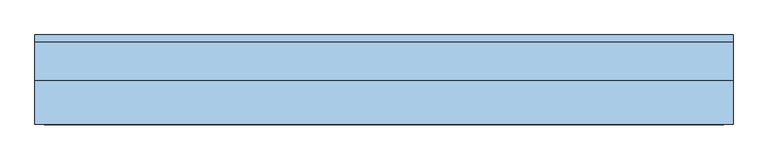
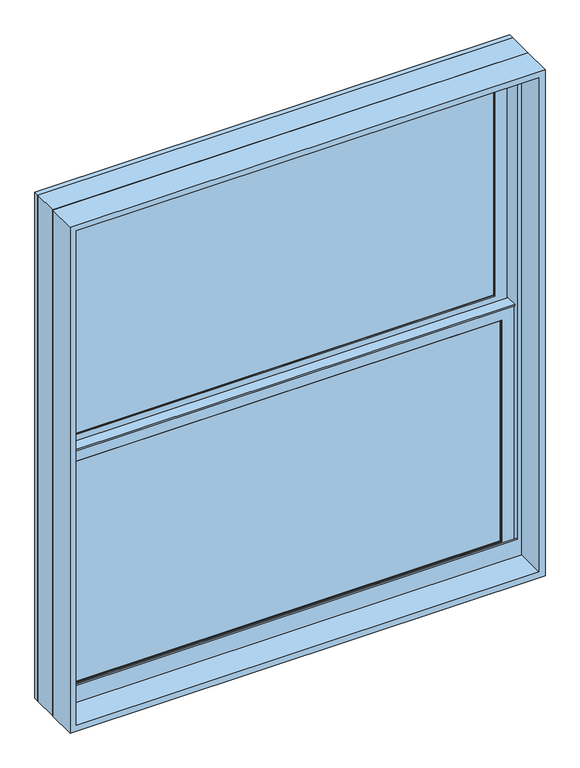
"""IFC4 building model written with IfcOpenShell, lengths in millimetres: window geometry, Window-Double_Hung-Marvin-Essential : ESDH4046."""

from ifc_helpers import new_model, si_unit, frame, origin, place, context, project, spatial, polyline, outline, extrude, faceted_brep, source, transform, mapped, element, save


def window_cdfb924c(model_context):
    return source(origin(), model_context, "Body", "SolidModel", [
        extrude(outline(polyline([(191.5583333, 20.6375), (191.5583333, 15.875), (172.5083333, 15.875), (172.5083333, 20.6375), (191.5583333, 20.6375)])), frame((0.0, 0.0, 1136.65), z_axis=(0.0, 0.0, 1.0), x_axis=(1.0, 0.0, 0.0)), (0.0, 0.0, 1.0), 603.25),
        extrude(outline(polyline([(-172.5083333, 20.6375), (-172.5083333, 15.875), (-191.5583333, 15.875), (-191.5583333, 20.6375), (-172.5083333, 20.6375)])), frame((0.0, 0.0, 1136.65), z_axis=(0.0, 0.0, 1.0), x_axis=(1.0, 0.0, 0.0)), (0.0, 0.0, 1.0), 603.25),
        extrude(outline(polyline([(546.1, 20.6375), (546.1, 15.875), (-546.1, 15.875), (-546.1, 20.6375), (546.1, 20.6375)])), frame((0.0, 0.0, 1428.75), z_axis=(0.0, 0.0, 1.0), x_axis=(1.0, 0.0, 0.0)), (0.0, 0.0, 1.0), 19.05),
        extrude(outline(polyline([(-191.5583333, 46.83125), (-191.5583333, 51.59375), (-172.5083333, 51.59375), (-172.5083333, 46.83125), (-191.5583333, 46.83125)])), frame((0.0, 0.0, 1778.0), z_axis=(0.0, 0.0, 1.0), x_axis=(1.0, 0.0, 0.0)), (0.0, 0.0, 1.0), 603.25),
        extrude(outline(polyline([(172.5083333, 46.83125), (172.5083333, 51.59375), (191.5583333, 51.59375), (191.5583333, 46.83125), (172.5083333, 46.83125)])), frame((0.0, 0.0, 1778.0), z_axis=(0.0, 0.0, 1.0), x_axis=(1.0, 0.0, 0.0)), (0.0, 0.0, 1.0), 603.25),
        extrude(outline(polyline([(-546.1, 46.83125), (-546.1, 51.59375), (546.1, 51.59375), (546.1, 46.83125), (-546.1, 46.83125)])), frame((0.0, 0.0, 2070.1), z_axis=(0.0, 0.0, 1.0), x_axis=(1.0, 0.0, 0.0)), (0.0, 0.0, 1.0), 19.05),
        extrude(outline(polyline([(191.5583333, 20.6375), (172.5083333, 20.6375), (172.5083333, 25.4), (191.5583333, 25.4), (191.5583333, 20.6375)])), frame((0.0, 0.0, 1136.65), z_axis=(0.0, 0.0, 1.0), x_axis=(1.0, 0.0, 0.0)), (0.0, 0.0, 1.0), 603.25),
        extrude(outline(polyline([(-172.5083333, 20.6375), (-191.5583333, 20.6375), (-191.5583333, 25.4), (-172.5083333, 25.4), (-172.5083333, 20.6375)])), frame((0.0, 0.0, 1136.65), z_axis=(0.0, 0.0, 1.0), x_axis=(1.0, 0.0, 0.0)), (0.0, 0.0, 1.0), 603.25),
        extrude(outline(polyline([(546.1, 20.6375), (-546.1, 20.6375), (-546.1, 25.4), (546.1, 25.4), (546.1, 20.6375)])), frame((0.0, 0.0, 1428.75), z_axis=(0.0, 0.0, 1.0), x_axis=(1.0, 0.0, 0.0)), (0.0, 0.0, 1.0), 19.05),
        extrude(outline(polyline([(-191.5583333, 56.35625), (-172.5083333, 56.35625), (-172.5083333, 51.59375), (-191.5583333, 51.59375), (-191.5583333, 56.35625)])), frame((0.0, 0.0, 1778.0), z_axis=(0.0, 0.0, 1.0), x_axis=(1.0, 0.0, 0.0)), (0.0, 0.0, 1.0), 603.25),
        extrude(outline(polyline([(172.5083333, 56.35625), (191.5583333, 56.35625), (191.5583333, 51.59375), (172.5083333, 51.59375), (172.5083333, 56.35625)])), frame((0.0, 0.0, 1778.0), z_axis=(0.0, 0.0, 1.0), x_axis=(1.0, 0.0, 0.0)), (0.0, 0.0, 1.0), 603.25),
        extrude(outline(polyline([(-546.1, 56.35625), (546.1, 56.35625), (546.1, 51.59375), (-546.1, 51.59375), (-546.1, 56.35625)])), frame((0.0, 0.0, 2070.1), z_axis=(0.0, 0.0, 1.0), x_axis=(1.0, 0.0, 0.0)), (0.0, 0.0, 1.0), 19.05),
        faceted_brep([(-573.0875, 5.6780605, 1769.9351748), (-573.0875, 5.6780605, 1765.3), (573.0875, 5.6780605, 1765.3), (573.0875, 5.6780605, 1769.9351748), (-573.0875, 34.8118605, 1769.9351748), (573.0875, 34.8118605, 1769.9351748), (573.0875, 34.8118605, 1765.3), (-573.0875, 34.8118605, 1765.3), (-573.0875, 30.1625, 1765.3), (-573.0875, 30.1625, 1109.6625), (-573.0875, 8.9241104, 1109.6625), (-573.0875, 8.9241104, 1765.3), (573.0875, 8.9241104, 1765.3), (573.0875, 30.1625, 1765.3), (573.0875, 8.9241104, 1109.6625), (573.0875, 30.1625, 1109.6625), (-557.2034752, 11.90625, 1751.0034752), (-557.2034752, 30.1625, 1751.0034752), (557.2034752, 30.1625, 1751.0034752), (557.2034752, 11.90625, 1751.0034752), (-540.54375, 10.4662439, 1734.34375), (-540.54375, 11.90625, 1734.34375), (540.54375, 11.90625, 1734.34375), (540.54375, 10.4662439, 1734.34375), (542.0858834, 8.9241104, 1735.8858834), (-542.0858834, 8.9241104, 1735.8858834), (557.2034752, 30.1625, 1125.5465248), (557.2034752, 11.90625, 1125.5465248), (540.54375, 11.90625, 1142.20625), (540.54375, 10.4662439, 1142.20625), (542.0858834, 8.9241104, 1140.6641166), (-557.2034752, 30.1625, 1125.5465248), (-557.2034752, 11.90625, 1125.5465248), (-540.54375, 11.90625, 1142.20625), (-540.54375, 10.4662439, 1142.20625), (-542.0858834, 8.9241104, 1140.6641166)], [[[0, 1, 2, 3]], [[4, 5, 6, 7]], [[1, 0, 4, 7, 8, 9, 10, 11]], [[2, 1, 11, 12]], [[7, 6, 13, 8]], [[3, 2, 12, 14, 15, 13, 6, 5]], [[0, 3, 5, 4]], [[16, 17, 18, 19]], [[20, 21, 22, 23]], [[20, 23, 24, 25]], [[19, 18, 26, 27]], [[23, 22, 28, 29]], [[24, 23, 29, 30]], [[27, 26, 31, 32]], [[29, 28, 33, 34]], [[30, 29, 34, 35]], [[15, 14, 10, 9]], [[15, 9, 8, 13], [18, 17, 31, 26]], [[17, 16, 32, 31]], [[16, 19, 27, 32], [22, 21, 33, 28]], [[21, 20, 34, 33]], [[20, 25, 35, 34]], [[10, 14, 12, 11], [25, 24, 30, 35]]]),
        extrude(outline(polyline([(38.5955581, 1751.0125), (33.5778968, 1751.0125), (33.5778968, 1752.6), (39.9405976, 1752.6), (39.9405976, 1751.0125), (61.515625, 1751.0125), (47.6307501, 1747.6975159), (38.5955581, 1747.6975159), (38.5955581, 1751.0125)])), frame((-573.0875, 0.0, 0.0), z_axis=(1.0, 0.0, 0.0), x_axis=(0.0, 1.0, 0.0)), (0.0, 0.0, 1.0), 1146.175),
        faceted_brep([(603.25, 0.0, 1079.5), (603.25, 0.0, 2438.4), (-603.25, 0.0, 2438.4), (-603.25, 0.0, 1079.5), (577.05625, 0.0, 1140.61875), (-577.05625, 0.0, 1140.61875), (-577.05625, 0.0, 2412.20625), (577.05625, 0.0, 2412.20625), (577.05625, 3.96875, 1079.5), (-577.05625, 3.96875, 1079.5), (-577.05625, 3.96875, 1140.61875), (577.05625, 3.96875, 1140.61875), (-603.25, 65.6828125, 1079.5), (-577.05625, 65.6828125, 1079.5), (577.05625, 65.6828125, 1079.5), (603.25, 65.6828125, 1079.5), (-603.25, 65.6828125, 2438.4), (603.25, 65.6828125, 2438.4), (577.05625, 65.6828125, 2412.20625), (-577.05625, 65.6828125, 2412.20625)], [[[0, 1, 2, 3], [4, 5, 6, 7]], [[8, 9, 10, 11]], [[5, 4, 11, 10]], [[0, 3, 12, 13, 9, 8, 14, 15]], [[13, 12, 16, 17, 15, 14, 18, 19]], [[13, 19, 6, 5, 10, 9]], [[7, 6, 19, 18]], [[18, 14, 8, 11, 4, 7]], [[1, 0, 15, 17]], [[2, 1, 17, 16]], [[3, 2, 16, 12]]]),
        faceted_brep([(577.05625, 30.1625, 1758.95), (575.46875, 30.1625, 1758.95), (575.46875, 30.1625, 1103.8544613), (577.05625, 30.1625, 1103.8544613), (-575.46875, 30.1625, 1758.95), (-577.05625, 30.1625, 1758.95), (-577.05625, 30.1625, 1103.8544613), (-575.46875, 30.1625, 1103.8544613), (575.46875, 63.5, 1758.95), (577.05625, 63.5, 1758.95), (577.05625, 63.5, 1097.3743077), (575.46875, 63.5, 1097.3743077), (-577.05625, 63.5, 1758.95), (-575.46875, 63.5, 1758.95), (-575.46875, 63.5, 1097.3743077), (-577.05625, 63.5, 1097.3743077), (588.3108932, 3.96875, 1108.9460105), (588.3108932, 3.96875, 1079.5), (588.3108932, 65.6828125, 1079.5), (588.3108932, 65.6828125, 1096.950012), (-588.3108932, 3.96875, 1079.5), (-588.3108932, 3.96875, 1108.9460105), (-588.3108932, 65.6828125, 1096.950012), (-588.3108932, 65.6828125, 1079.5), (588.3108932, 78.58125, 1094.4428097), (-588.3108932, 78.58125, 1094.4428097), (-586.2971252, 68.2348864, 1096.4539391), (-568.33135, 68.2348864, 1096.4539391), (-568.33135, 65.6828125, 1096.950012), (568.33135, 65.6828125, 1096.950012), (568.33135, 68.2348864, 1096.4539391), (586.2971252, 68.2348864, 1096.4539391), (-603.25, 65.6828125, 1079.5), (-603.25, 78.5948249, 1079.5), (603.25, 78.5948249, 1079.5), (603.25, 65.6828125, 1079.5), (-603.25, 78.58125, 2438.4), (603.25, 78.58125, 2438.4), (588.3108932, 78.58125, 2423.4608932), (-588.3108932, 78.58125, 2423.4608932), (-603.25, 65.6828125, 2438.4), (-586.2971252, 68.2348864, 2421.4471252), (586.2971252, 68.2348864, 2421.4471252), (568.33135, 68.2348864, 2403.48135), (-568.33135, 68.2348864, 2403.48135), (-568.33135, 65.6828125, 2403.48135), (568.33135, 65.6828125, 2403.48135), (603.25, 65.6828125, 2438.4)], [[[0, 1, 2, 3]], [[4, 5, 6, 7]], [[8, 9, 10, 11]], [[12, 13, 14, 15]], [[1, 8, 11, 2]], [[9, 0, 3, 10]], [[1, 0, 9, 8]], [[5, 4, 13, 12]], [[5, 12, 15, 6]], [[13, 4, 7, 14]], [[16, 17, 18, 19]], [[20, 21, 22, 23]], [[24, 25, 26, 27, 28, 22, 21, 16, 19, 29, 30, 31], [3, 2, 11, 10], [7, 6, 15, 14]], [[17, 16, 21, 20]], [[17, 20, 23, 32, 33, 34, 35, 18]], [[34, 33, 36, 37], [25, 24, 38, 39]], [[33, 32, 40, 36]], [[39, 41, 26, 25]], [[41, 42, 31, 30, 43, 44, 27, 26]], [[44, 45, 28, 27]], [[40, 32, 23, 22, 28, 45, 46, 29, 19, 18, 35, 47]], [[36, 40, 47, 37]], [[39, 38, 42, 41]], [[44, 43, 46, 45]], [[34, 37, 47, 35]], [[42, 38, 24, 31]], [[46, 43, 30, 29]]]),
        extrude(outline(polyline([(553.24375, 11.90625), (-553.24375, 11.90625), (-553.24375, 15.08125), (553.24375, 15.08125), (553.24375, 11.90625)])), frame((0.0, 0.0, 1129.50625), z_axis=(0.0, 0.0, 1.0), x_axis=(1.0, 0.0, 0.0)), (0.0, 0.0, 1.0), 617.5375),
        extrude(outline(polyline([(553.24375, 42.8625), (-553.24375, 42.8625), (-553.24375, 46.0375), (553.24375, 46.0375), (553.24375, 42.8625)])), frame((0.0, 0.0, 1770.85625), z_axis=(0.0, 0.0, 1.0), x_axis=(1.0, 0.0, 0.0)), (0.0, 0.0, 1.0), 617.5375),
        faceted_brep([(-540.54375, 31.194477, 1734.34375), (-542.0858834, 32.7366104, 1735.8858834), (542.0858834, 32.7366104, 1735.8858834), (540.54375, 31.194477, 1734.34375), (-540.54375, 30.1625, 1734.34375), (540.54375, 30.1625, 1734.34375), (-573.0875, 32.7366104, 1766.8875), (-573.0875, 30.1625, 1766.8875), (573.0875, 30.1625, 1766.8875), (573.0875, 32.7366104, 1766.8875), (542.0858834, 32.7366104, 1140.6641166), (540.54375, 31.194477, 1142.20625), (540.54375, 30.1625, 1142.20625), (573.0875, 30.1625, 1109.6625), (573.0875, 32.7366104, 1109.6625), (-542.0858834, 32.7366104, 1140.6641166), (-540.54375, 31.194477, 1142.20625), (-540.54375, 30.1625, 1142.20625), (-573.0875, 30.1625, 1109.6625), (-573.0875, 32.7366104, 1109.6625)], [[[0, 1, 2, 3]], [[4, 0, 3, 5]], [[6, 7, 8, 9]], [[3, 2, 10, 11]], [[5, 3, 11, 12]], [[9, 8, 13, 14]], [[11, 10, 15, 16]], [[12, 11, 16, 17]], [[14, 13, 18, 19]], [[9, 14, 19, 6], [1, 15, 10, 2]], [[16, 15, 1, 0]], [[17, 16, 0, 4]], [[7, 18, 13, 8], [5, 12, 17, 4]], [[19, 18, 7, 6]]]),
        faceted_brep([(-557.2034752, 42.8625, 2392.3534752), (-557.2034752, 61.11875, 2392.3534752), (557.2034752, 61.11875, 2392.3534752), (557.2034752, 42.8625, 2392.3534752), (-540.54375, 41.4224939, 2375.69375), (-540.54375, 42.8625, 2375.69375), (540.54375, 42.8625, 2375.69375), (540.54375, 41.4224939, 2375.69375), (-542.0858834, 39.8803604, 2377.2358834), (542.0858834, 39.8803604, 2377.2358834), (-573.0875, 61.11875, 2408.2375), (-573.0875, 39.8803604, 2408.2375), (573.0875, 39.8803604, 2408.2375), (573.0875, 61.11875, 2408.2375), (557.2034752, 61.11875, 1766.8965248), (557.2034752, 42.8625, 1766.8965248), (540.54375, 42.8625, 1783.55625), (540.54375, 41.4224939, 1783.55625), (542.0858834, 39.8803604, 1782.0141166), (573.0875, 39.8803604, 1751.0125), (573.0875, 61.11875, 1751.0125), (-557.2034752, 61.11875, 1766.8965248), (-557.2034752, 42.8625, 1766.8965248), (-540.54375, 42.8625, 1783.55625), (-540.54375, 41.4224939, 1783.55625), (-542.0858834, 39.8803604, 1782.0141166), (-573.0875, 39.8803604, 1751.0125), (-573.0875, 61.11875, 1751.0125)], [[[0, 1, 2, 3]], [[4, 5, 6, 7]], [[8, 4, 7, 9]], [[10, 11, 12, 13]], [[3, 2, 14, 15]], [[7, 6, 16, 17]], [[9, 7, 17, 18]], [[13, 12, 19, 20]], [[15, 14, 21, 22]], [[17, 16, 23, 24]], [[18, 17, 24, 25]], [[20, 19, 26, 27]], [[13, 20, 27, 10], [1, 21, 14, 2]], [[22, 21, 1, 0]], [[3, 15, 22, 0], [5, 23, 16, 6]], [[24, 23, 5, 4]], [[25, 24, 4, 8]], [[11, 26, 19, 12], [9, 18, 25, 8]], [[27, 26, 11, 10]]]),
        faceted_brep([(-573.0875, 61.11875, 1751.0125), (-573.0875, 63.6928604, 1751.0125), (573.0875, 63.6928604, 1751.0125), (573.0875, 61.11875, 1751.0125), (-540.54375, 62.150727, 1783.55625), (-540.54375, 61.11875, 1783.55625), (540.54375, 61.11875, 1783.55625), (540.54375, 62.150727, 1783.55625), (-542.0858834, 63.6928604, 1782.0141166), (542.0858834, 63.6928604, 1782.0141166), (573.0875, 63.6928604, 2408.2375), (573.0875, 61.11875, 2408.2375), (540.54375, 61.11875, 2375.69375), (540.54375, 62.150727, 2375.69375), (542.0858834, 63.6928604, 2377.2358834), (-573.0875, 63.6928604, 2408.2375), (-573.0875, 61.11875, 2408.2375), (-540.54375, 61.11875, 2375.69375), (-540.54375, 62.150727, 2375.69375), (-542.0858834, 63.6928604, 2377.2358834)], [[[0, 1, 2, 3]], [[4, 5, 6, 7]], [[8, 4, 7, 9]], [[3, 2, 10, 11]], [[7, 6, 12, 13]], [[9, 7, 13, 14]], [[11, 10, 15, 16]], [[13, 12, 17, 18]], [[14, 13, 18, 19]], [[16, 15, 1, 0]], [[3, 11, 16, 0], [5, 17, 12, 6]], [[18, 17, 5, 4]], [[19, 18, 4, 8]], [[1, 15, 10, 2], [9, 14, 19, 8]]]),
        extrude(outline(polyline([(553.24375, 26.19375), (-553.24375, 26.19375), (-553.24375, 30.1625), (553.24375, 30.1625), (553.24375, 26.19375)])), frame((0.0, 0.0, 1129.50625), z_axis=(0.0, 0.0, 1.0), x_axis=(1.0, 0.0, 0.0)), (0.0, 0.0, 1.0), 617.5375),
        extrude(outline(polyline([(553.24375, 57.15), (-553.24375, 57.15), (-553.24375, 61.11875), (553.24375, 61.11875), (553.24375, 57.15)])), frame((0.0, 0.0, 1770.85625), z_axis=(0.0, 0.0, 1.0), x_axis=(1.0, 0.0, 0.0)), (0.0, 0.0, 1.0), 617.5375),
        extrude(outline(polyline([(2438.4, 603.25), (2438.4, -603.25), (1079.5, -603.25), (1079.5, 603.25), (2438.4, 603.25)]), holes=[polyline([(2422.525, 587.375), (1095.375, 587.375), (1095.375, -587.375), (2422.525, -587.375), (2422.525, 587.375)])]), frame((0.0, -76.2, 0.0), z_axis=(0.0, 1.0, 0.0), x_axis=(0.0, 0.0, 1.0)), (0.0, 0.0, 1.0), 75.40625),
    ])


if __name__ == "__main__":
    model = new_model("IFC4")
    model_context = context("Model", 3, world=origin())
    ifc_project = project(units=[si_unit("LENGTHUNIT", "METRE", prefix="MILLI")], contexts=[model_context])
    site = spatial("IfcSite", under=ifc_project)
    building = spatial("IfcBuilding", under=site)
    placement = place(None, origin())
    window_shape = window_cdfb924c(model_context)
    element("IfcWindow", 1, ObjectType="Window-Double_Hung-Marvin-Essential : ESDH4046", at=placement, inside=building, context=model_context, shape_type="MappedRepresentation", body=[
        mapped(window_shape, transform((0.0, 0.0, 0.0), x_axis=(1.0, 0.0, 0.0), y_axis=(0.0, 1.0, 0.0), z_axis=(0.0, 0.0, 1.0))),
    ])
    save(model, "model.ifc")

# Revit data of these elements
# Type "Window-Double_Hung-Marvin-Essential : ESDH4046"
#   Type Mark = "60"
#   Window Type = "Essential Double Hung"
#   Product data url = "https://bimobject.com/marvin-windows-and-doors/product/marvin-dhwau"
#   Product Guid = "c4a96547-874c-4385-91dc-a058adc19d98"
#   Frame = "All Ultrex"
#   Egress Window = "No"
#   URL = "www.marvin.com"
#   Model = "ESDH4046"
#   Manufacturer = "Marvin Windows and Doors"
#   Label Egress = ""
#   Glass Type = "IG Low E II with Argon"
#   Design Pressure = "DP40"
#   Description = "4854 DBHG"
#   Analytic Construction = "<None>"
#   Prairie Corner Width = 0' - 4"
#   Prairie Corner Height = 0' - 4"
#   Egress Width = 3' - 8 9/16"
#   Egress Height = 1' - 10 27/128"
#   Rough Width = 4' - 0"
#   Rough Height = 4' - 6"
#   Nominal Width = 4' - 0"
#   Nominal Height = 4' - 6"
#   Inset to Installation Flange [instance default] = 0' - 1"
#   Height = 4' - 5 1/2"
#   Egress Area = 6.87344 SF
#   Default Head Height = 8' - 0"
#   Width = 3' - 11 1/2"
#   Daylight Area = 13.7811 SF
#   DLO Width = 3' - 6 9/16"
#   DLO Height = 1' - 11 5/16"
#   Muntins Top Sash = yes
#   Lites Wide Top Sash = 3
#   Lites Wide Bottom Sash = 3
#   Lites High Top Sash = 2
#   Lites High Bottom Sash = 2
#   Lite Cut Prairie 9 = no
#   Lite Cut HV Grid = yes
#   Muntins Bottom Sash = yes
#   Label Visibility = no
#   Jamb Extension Visibility = yes
#   Edition number = 1
#   Interior Material = Ultrex-Marvin-Stonewhite
#   Glazing Material = Glass-Marvin-IG Low E II with Argon
#   Cladding Material = Ultrex-Marvin-Pebblegray
#   Wall Closure = (empty or 0)
#   Assembly Code = ""
# Element 1 (IfcWindow, "Window-Double_Hung-Marvin-Essential : ESDH4046")
#   Materials on its faces: "Ultrex-Marvin-Pebblegray", "Ultrex-Marvin-Stonewhite", "Glass-Marvin-IG Low E II with Argon"
# Materials
#   "Ultrex-Marvin-Stonewhite": class "Paint", colour RGB 250 251 245, transparency 0
#   "Glass-Marvin-IG Low E II with Argon": class "Glass", colour RGB 0 128 192, transparency 0.85
#   "Ultrex-Marvin-Pebblegray": class "Paint", colour RGB 189 185 173, transparency 0
